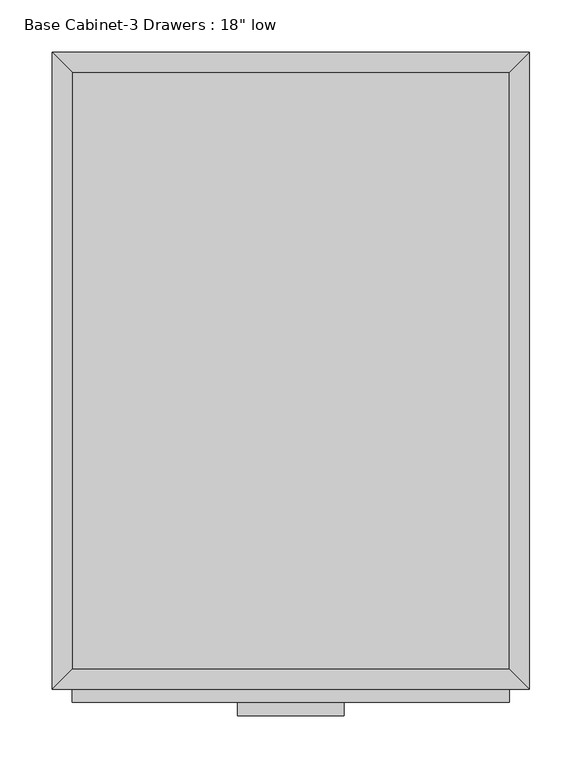
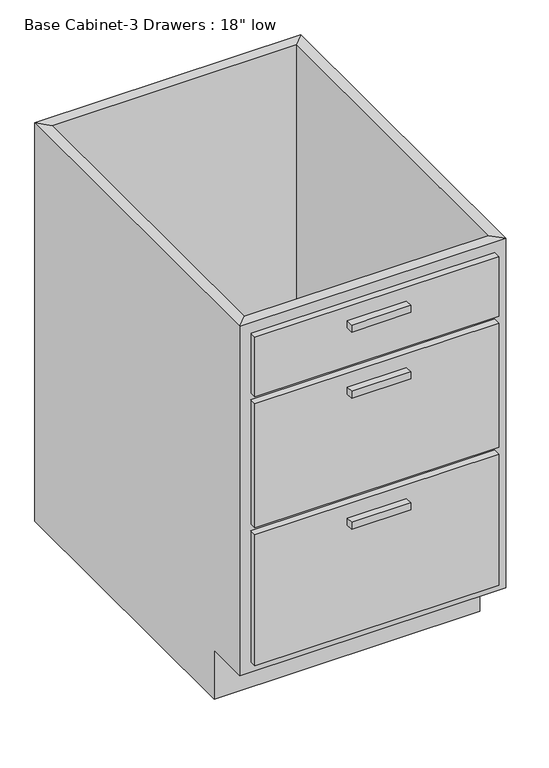
"""IFC4 building model written with IfcOpenShell, lengths in millimetres: furniture geometry."""

import ifcopenshell
import ifcopenshell.guid

model = None  # the IFC model being written
_history = None  # IfcOwnerHistory: only IFC2X3 demands one
_inside = {}  # id of a spatial element -> (the spatial element, [elements in it])
_under = {}  # id of a project, library or spatial element -> (it, [spatial elements below it])
_declared = {}  # id of a project -> (the project, [libraries it declares])
_typed = {}  # id of a type object -> (the type object, [elements of that type])
_made_of = {}  # id of a material, layer set ... -> (it, [elements and type objects made of it])


def new_model(schema):
    """Start an empty IFC model of exactly this schema.

    Asked for "IFC4X3", IfcOpenShell would pick the latest addendum, in which some entities
    have other attributes; the version numbers below select the first issue.
    IFC2X3 requires an IfcOwnerHistory on every rooted entity: one is made here for all.
    """
    global model, _history
    if schema == "IFC4X3":
        model = ifcopenshell.file(schema_version=(4, 3, 0, 0))
    else:
        model = ifcopenshell.file(schema=schema)
    _inside.clear()
    _under.clear()
    _declared.clear()
    _typed.clear()
    _made_of.clear()
    _history = None
    if model.schema == "IFC2X3":
        org = make("IfcOrganization", Name="unknown")
        user = make(
            "IfcPersonAndOrganization",
            ThePerson=make("IfcPerson", FamilyName="unknown"),
            TheOrganization=org,
        )
        app = make(
            "IfcApplication",
            ApplicationDeveloper=org,
            Version="unknown",
            ApplicationFullName="unknown",
            ApplicationIdentifier="unknown",
        )
        _history = make(
            "IfcOwnerHistory",
            OwningUser=user,
            OwningApplication=app,
            ChangeAction="ADDED",
            CreationDate=0,
        )
    return model


def make(cls, **values):
    """One entity of the class cls with the attributes given. An attribute that is None is left unset."""
    return model.create_entity(
        cls, **{name: value for name, value in values.items() if value is not None}
    )


def rooted(cls, **values):
    """An entity with a GlobalId (a new one), such as an element, a storey or a relation."""
    return make(cls, GlobalId=ifcopenshell.guid.new(), OwnerHistory=_history, **values)


def si_unit(unit_type, name, prefix=None):
    """IfcSIUnit, for example si_unit("LENGTHUNIT", "METRE", prefix="MILLI")."""
    return make("IfcSIUnit", UnitType=unit_type, Prefix=prefix, Name=name)


def assignment(units):
    """IfcUnitAssignment: the units of a project."""
    return None if units is None else make("IfcUnitAssignment", Units=units)


def point(xyz):
    """IfcCartesianPoint."""
    return None if xyz is None else make("IfcCartesianPoint", Coordinates=xyz)


def direction(xyz):
    """IfcDirection."""
    return None if xyz is None else make("IfcDirection", DirectionRatios=xyz)


def frame(location, z_axis=None, x_axis=None):
    """IfcAxis2Placement3D, a coordinate frame: its origin and axes. An axis left out is left unset."""
    return make(
        "IfcAxis2Placement3D",
        Location=point(location),
        Axis=direction(z_axis),
        RefDirection=direction(x_axis),
    )


def origin():
    """The frame at (0, 0, 0) with its axes left unset."""
    return frame((0.0, 0.0, 0.0))


def place(relative_to, where):
    """IfcLocalPlacement: puts the frame where relative to a parent placement (None: the world)."""
    return make(
        "IfcLocalPlacement", PlacementRelTo=relative_to, RelativePlacement=where
    )


def context(
    kind, dimensions, precision=None, world=None, true_north=None, identifier=None
):
    """IfcGeometricRepresentationContext, for example the 3D "Model" context."""
    return make(
        "IfcGeometricRepresentationContext",
        ContextIdentifier=identifier,
        ContextType=kind,
        CoordinateSpaceDimension=dimensions,
        Precision=precision,
        WorldCoordinateSystem=world,
        TrueNorth=true_north,
    )


def project(units=None, contexts=None):
    """IfcProject with its units and contexts."""
    return rooted(
        "IfcProject",
        Name="project",
        RepresentationContexts=contexts,
        UnitsInContext=assignment(units),
    )


def spatial(cls, under=None, at=None, **own):
    """A site, building, storey or space (cls), placed at a placement, below another one or the project."""
    s = rooted(cls, ObjectPlacement=at, **own)
    if under is not None:
        _under.setdefault(under.id(), (under, []))[1].append(s)
    return s


def polyline(points):
    """IfcPolyline through the points."""
    return make("IfcPolyline", Points=[point(p) for p in points])


def outline(outer, holes=None, kind="AREA"):
    """IfcArbitraryClosedProfileDef: a profile drawn as a closed curve; with holes, ...WithVoids."""
    if holes is None:
        return make("IfcArbitraryClosedProfileDef", ProfileType=kind, OuterCurve=outer)
    return make(
        "IfcArbitraryProfileDefWithVoids",
        ProfileType=kind,
        OuterCurve=outer,
        InnerCurves=holes,
    )


def extrude(swept, where, along, depth):
    """IfcExtrudedAreaSolid: the profile swept, set in the frame where, extruded along a direction by depth."""
    return make(
        "IfcExtrudedAreaSolid",
        SweptArea=swept,
        Position=where,
        ExtrudedDirection=direction(along),
        Depth=depth,
    )


def faces_of(points, faces, orient=None, outer=None):
    """IfcFace entities. A face is a list of loops; a loop is a list of indices into points, from 0.

    orient and outer hold one flag for each loop. By default every Orientation is true, the
    first loop of a face is its IfcFaceOuterBound and the others are IfcFaceBound.
    """
    made = []
    for i, loops in enumerate(faces):
        bounds = []
        for j, loop in enumerate(loops):
            is_outer = j == 0 if outer is None else outer[i][j]
            bounds.append(
                make(
                    "IfcFaceOuterBound" if is_outer else "IfcFaceBound",
                    Bound=make("IfcPolyLoop", Polygon=[points[k] for k in loop]),
                    Orientation=True if orient is None else orient[i][j],
                )
            )
        made.append(make("IfcFace", Bounds=bounds))
    return made


def faceted_brep(points, faces, orient=None, outer=None, voids=None):
    """IfcFacetedBrep: a solid bounded by flat faces; with voids (closed shells), ...WithVoids."""
    shared = [point(p) for p in points]
    hull = make("IfcClosedShell", CfsFaces=faces_of(shared, faces, orient, outer))
    if voids is None:
        return make("IfcFacetedBrep", Outer=hull)
    return make(
        "IfcFacetedBrepWithVoids",
        Outer=hull,
        Voids=[
            make(cls, CfsFaces=faces_of(shared, fs, o, b)) for cls, fs, o, b in voids
        ],
    )


def shape(context_of_items, identifier, shape_type, items):
    """IfcShapeRepresentation: the items that make up one representation, for example the "Body"."""
    return make(
        "IfcShapeRepresentation",
        ContextOfItems=context_of_items,
        RepresentationIdentifier=identifier,
        RepresentationType=shape_type,
        Items=items,
    )


def source(mapping_origin, context_of_items, identifier, shape_type, items):
    """IfcRepresentationMap: a shape defined once, which mapped items show again and again."""
    return make(
        "IfcRepresentationMap",
        MappingOrigin=mapping_origin,
        MappedRepresentation=shape(context_of_items, identifier, shape_type, items),
    )


def transform(
    local_origin,
    x_axis=None,
    y_axis=None,
    z_axis=None,
    scale=None,
    scale2=None,
    scale3=None,
    uniform=True,
):
    """IfcCartesianTransformationOperator3D, or its non-uniform kind. x_axis, y_axis, z_axis: its Axis1, 2, 3."""
    if uniform:
        return make(
            "IfcCartesianTransformationOperator3D",
            Axis1=direction(x_axis),
            Axis2=direction(y_axis),
            LocalOrigin=point(local_origin),
            Scale=scale,
            Axis3=direction(z_axis),
        )
    return make(
        "IfcCartesianTransformationOperator3DnonUniform",
        Axis1=direction(x_axis),
        Axis2=direction(y_axis),
        LocalOrigin=point(local_origin),
        Scale=scale,
        Axis3=direction(z_axis),
        Scale2=scale2,
        Scale3=scale3,
    )


def mapped(mapping_source, mapping_target):
    """IfcMappedItem: shows the shape of a source again, moved by a transform."""
    return make(
        "IfcMappedItem", MappingSource=mapping_source, MappingTarget=mapping_target
    )


def made_of(thing, what):
    """Note that an element or type object is made of a material, layer set ...; save() writes the relation."""
    if what is not None:
        _made_of.setdefault(what.id(), (what, []))[1].append(thing)
    return thing


def element(
    cls,
    number,
    at=None,
    inside=None,
    cuts=None,
    type_object=None,
    material=None,
    context=None,
    identifier="Body",
    shape_type=None,
    held_by="IfcProductDefinitionShape",
    body=None,
    shapes=None,
    **own,
):
    """One element of the class cls, such as IfcWall. Its Tag is "e" and its number.

    at: its placement. inside: the storey or other place that contains it. cuts: it is an
    opening in that element (IfcRelVoidsElement). A single representation is given by context,
    identifier, shape_type and body (its items); several are given by shapes. held_by: the class
    of the entity that holds the representations. save() writes the other relations.
    """
    e = rooted(cls, Tag="e%d" % number, ObjectPlacement=at, **own)
    if body is not None:
        shapes = [shape(context, identifier, shape_type, body)]
    if shapes is not None:
        e.Representation = make(held_by, Representations=shapes)
    if inside is not None:
        _inside.setdefault(inside.id(), (inside, []))[1].append(e)
    if cuts is not None:
        rooted(
            "IfcRelVoidsElement", RelatingBuildingElement=cuts, RelatedOpeningElement=e
        )
    if type_object is not None:
        _typed.setdefault(type_object.id(), (type_object, []))[1].append(e)
    return made_of(e, material)


def aggregate(whole, parts):
    """IfcRelAggregates: a whole, such as a stair, and the parts it consists of."""
    return rooted("IfcRelAggregates", RelatingObject=whole, RelatedObjects=parts)


def save(model, path):
    """Write the relations noted so far, then the file.

    IfcRelAggregates (storeys below a building ...), IfcRelContainedInSpatialStructure (elements
    in a storey), IfcRelDefinesByType, IfcRelAssociatesMaterial and IfcRelDeclares: one each for
    every whole, place, type object, material and project.
    """
    for whole, parts in _under.values():
        aggregate(whole, parts)
    for where, things in _inside.values():
        rooted(
            "IfcRelContainedInSpatialStructure",
            RelatedElements=things,
            RelatingStructure=where,
        )
    for kind, things in _typed.values():
        rooted("IfcRelDefinesByType", RelatedObjects=things, RelatingType=kind)
    for what, things in _made_of.values():
        rooted("IfcRelAssociatesMaterial", RelatedObjects=things, RelatingMaterial=what)
    for by, libraries in _declared.values():
        rooted("IfcRelDeclares", RelatingContext=by, RelatedDefinitions=libraries)
    model.write(path)


def furniture_8bab169b(model_context):
    return source(origin(), model_context, "Body", "SolidModel", [
        faceted_brep([(-190.8122951, -533.4, 88.9), (228.2877049, -533.4, 88.9), (228.2877049, -19.05, 88.9), (-190.8122951, -19.05, 88.9), (247.3377049, 0.0, 0.0), (247.3377049, -533.4, 0.0), (-209.8622951, -533.4, 0.0), (-209.8622951, 0.0, 0.0), (-209.8622951, 0.0, 723.9), (247.3377049, 0.0, 723.9), (-209.8622951, -533.4, 88.9), (-209.8622951, -609.6, 88.9), (-209.8622951, -609.6, 723.9), (247.3377049, -533.4, 88.9), (247.3377049, -609.6, 723.9), (247.3377049, -609.6, 88.9), (228.2877049, -590.55, 723.9), (228.2877049, -590.55, 88.9), (-190.8122951, -590.55, 88.9), (-190.8122951, -590.55, 723.9), (-190.8122951, -19.05, 723.9), (228.2877049, -19.05, 723.9)], [[[0, 1, 2, 3]], [[4, 5, 6, 7]], [[4, 7, 8, 9]], [[8, 7, 6, 10, 11, 12]], [[6, 5, 13, 1, 0, 10]], [[5, 4, 9, 14, 15, 13]], [[16, 17, 18, 19]], [[16, 19, 12, 14]], [[14, 12, 11, 15]], [[18, 17, 15, 11]], [[19, 18, 0, 3, 20]], [[12, 19, 20, 8]], [[18, 11, 10, 0]], [[20, 3, 2, 21]], [[8, 20, 21, 9]], [[17, 16, 21, 2, 1]], [[16, 14, 9, 21]], [[15, 17, 1, 13]]]),
        extrude(outline(polyline([(69.5377049, -635.0), (-32.0622951, -635.0), (-32.0622951, -622.3), (69.5377049, -622.3), (69.5377049, -635.0)])), frame((0.0, 0.0, 666.75), z_axis=(0.0, 0.0, 1.0), x_axis=(1.0, 0.0, 0.0)), (0.0, 0.0, 1.0), 12.7),
        extrude(outline(polyline([(69.5377049, -635.0), (-32.0622951, -635.0), (-32.0622951, -622.3), (69.5377049, -622.3), (69.5377049, -635.0)])), frame((0.0, 0.0, 546.1), z_axis=(0.0, 0.0, 1.0), x_axis=(1.0, 0.0, 0.0)), (0.0, 0.0, 1.0), 12.7),
        extrude(outline(polyline([(69.5377049, -635.0), (-32.0622951, -635.0), (-32.0622951, -622.3), (69.5377049, -622.3), (69.5377049, -635.0)])), frame((0.0, 0.0, 307.975), z_axis=(0.0, 0.0, 1.0), x_axis=(1.0, 0.0, 0.0)), (0.0, 0.0, 1.0), 12.7),
        extrude(outline(polyline([(228.2877049, -622.3), (-190.8122951, -622.3), (-190.8122951, -609.6), (228.2877049, -609.6), (228.2877049, -622.3)])), frame((0.0, 0.0, 596.9), z_axis=(0.0, 0.0, 1.0), x_axis=(1.0, 0.0, 0.0)), (0.0, 0.0, 1.0), 107.95),
        extrude(outline(polyline([(228.2877049, -622.3), (-190.8122951, -622.3), (-190.8122951, -609.6), (228.2877049, -609.6), (228.2877049, -622.3)])), frame((0.0, 0.0, 358.775), z_axis=(0.0, 0.0, 1.0), x_axis=(1.0, 0.0, 0.0)), (0.0, 0.0, 1.0), 225.425),
        extrude(outline(polyline([(228.2877049, -622.3), (-190.8122951, -622.3), (-190.8122951, -609.6), (228.2877049, -609.6), (228.2877049, -622.3)])), frame((0.0, 0.0, 107.95), z_axis=(0.0, 0.0, 1.0), x_axis=(1.0, 0.0, 0.0)), (0.0, 0.0, 1.0), 238.125),
        extrude(outline(polyline([(228.2877049, -19.05), (228.2877049, -590.55), (-190.8122951, -590.55), (-190.8122951, -19.05), (228.2877049, -19.05)])), frame((0.0, 0.0, 88.9), z_axis=(0.0, 0.0, 1.0), x_axis=(1.0, 0.0, 0.0)), (0.0, 0.0, 1.0), 19.05),
    ])


if __name__ == "__main__":
    model = new_model("IFC4")
    model_context = context("Model", 3, world=origin())
    ifc_project = project(units=[si_unit("LENGTHUNIT", "METRE", prefix="MILLI")], contexts=[model_context])
    site = spatial("IfcSite", under=ifc_project)
    building = spatial("IfcBuilding", under=site)
    placement = place(None, origin())
    furniture_shape = furniture_8bab169b(model_context)
    element("IfcFurniture", 1, ObjectType="Base Cabinet-3 Drawers : 18\" low", at=placement, inside=building, context=model_context, shape_type="MappedRepresentation", body=[
        mapped(furniture_shape, transform((0.0, 0.0, 0.0), x_axis=(1.0, 0.0, 0.0), y_axis=(0.0, 1.0, 0.0), z_axis=(0.0, 0.0, 1.0))),
    ])
    save(model, "model.ifc")

# Revit data of these elements
# Type "Base Cabinet-3 Drawers : 18\" low"
#   Assembly Code = "C1030410"
#   Depth = 2' - 0"
#   Height = 2' - 4 1/2"
#   Toe Depth = 0' - 3"
#   Toe Height = 0' - 3 1/2"
#   Width = 1' - 6"
#   Handle Material = Cabinets - Handles
#   Door/Drawer Material = Cabinets
#   Cabinet Material = Cabinets
#   Default Elevation = 0
# Element 1 (IfcFurniture, "Base Cabinet-3 Drawers : 18\" low")
#   Materials on its faces: "Cabinets", "Cabinets - Handles"
# Materials
#   "Cabinets - Handles": class "Unassigned", colour RGB 57 57 57, transparency 0
#   "Cabinets": class "Unassigned", colour RGB 249 249 249, transparency 0
